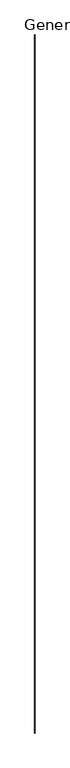
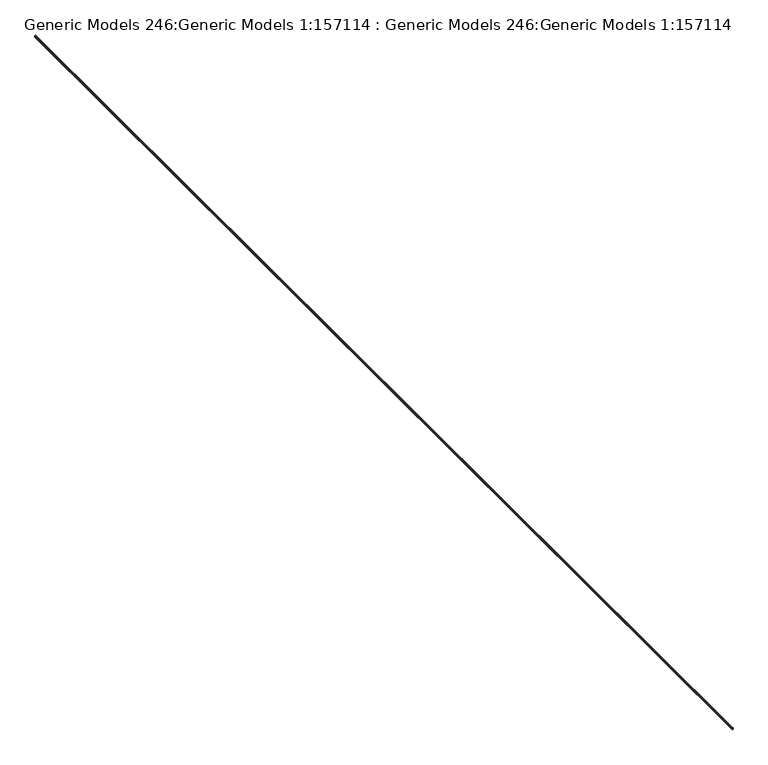
"""IFC4 building model written with IfcOpenShell, lengths in millimetres: proxy geometry, Generic Models 246:Generic Models 1:157114 : Generic Models 246:Generic Models 1:157114."""

from ifc_helpers import new_model, si_unit, point, frame, frame_2d, origin, place, context, project, spatial, polyline, circle_curve, trimmed, segment, composite_curve, outline, extrude, source, transform, mapped, element, save


def generic_models_246_generic_models_1_157114_generic_models_ae619eab(model_context):
    return source(origin(), model_context, "Body", "SweptSolid", [
        extrude(outline(composite_curve([segment(trimmed(circle_curve(frame_2d((6034.2282742, 2076.0989222)), 4.3100275), [point((6037.1430147, 2072.9239222))], [point((6037.1430147, 2079.2739222))], True, "CARTESIAN"), True, "CONTINUOUS"), segment(polyline([(6037.1430147, 2079.2739222), (6040.3180147, 2079.2739222)]), True, "CONTINUOUS"), segment(trimmed(circle_curve(frame_2d((6037.4032742, 2076.0989222)), 4.3100275), [point((6040.3180147, 2079.2739222))], [point((6041.269774, 2078.0032636))], False, "CARTESIAN"), True, "CONTINUOUS"), segment(polyline([(6041.269774, 2078.0032636), (6041.9750492, 2078.5060865), (6042.8263165, 2078.8957455), (6043.7835566, 2079.1539221), (6044.8017683, 2079.2684792), (6045.8330843, 2079.2340312), (6046.829021, 2079.0521977), (6047.7427582, 2078.7315268), (6048.5313398, 2078.2870936), (6049.1576935, 2077.7397917), (6049.8149455, 2075.7547189), (6049.1576935, 2074.4580526), (6048.5313398, 2073.9107507), (6047.7427582, 2073.4663175), (6046.829021, 2073.1456466), (6045.8330843, 2072.9638131), (6044.8017683, 2072.9293651), (6043.7835566, 2073.0439222), (6042.8263165, 2073.3020988), (6041.9750492, 2073.6917578), (6041.269774, 2074.1945807)]), True, "CONTINUOUS"), segment(trimmed(circle_curve(frame_2d((6037.4032742, 2076.0989222)), 4.3100275), [point((6041.269774, 2074.1945807))], [point((6040.3180147, 2072.9239222))], False, "CARTESIAN"), True, "CONTINUOUS"), segment(polyline([(6040.3180147, 2072.9239222), (6037.1430147, 2072.9239222)]), True, "CONTINUOUS")], self_intersect=False)), frame((0.0, 496.8218843, 0.0), z_axis=(0.0, 1.0, 0.0), x_axis=(0.0, 0.0, 1.0)), (0.0, 0.0, 1.0), 7886.7),
    ])


if __name__ == "__main__":
    model = new_model("IFC4")
    model_context = context("Model", 3, world=origin())
    ifc_project = project(units=[si_unit("LENGTHUNIT", "METRE", prefix="MILLI")], contexts=[model_context])
    site = spatial("IfcSite", under=ifc_project)
    building = spatial("IfcBuilding", under=site)
    placement = place(None, origin())
    generic_models_246_generic_models_1_157114_generic_models_shape = generic_models_246_generic_models_1_157114_generic_models_ae619eab(model_context)
    element("IfcBuildingElementProxy", 1, Name="Generic Models 246:Generic Models 1:157114 : Generic Models 246:Generic Models 1:157114", ObjectType="Generic Models 246:Generic Models 1:157114 : Generic Models 246:Generic Models 1:157114", at=placement, inside=building, context=model_context, shape_type="MappedRepresentation", body=[
        mapped(generic_models_246_generic_models_1_157114_generic_models_shape, transform((0.0, 0.0, 0.0), x_axis=(1.0, 0.0, 0.0), y_axis=(0.0, 1.0, 0.0), z_axis=(0.0, 0.0, 1.0))),
    ])
    save(model, "model.ifc")

# Revit data of these elements
# Type "Generic Models 246:Generic Models 1:157114 : Generic Models 246:Generic Models 1:157114"
#   NameOverride = "Generic Models 246:Generic Models 1:157114"
#   ObjectTypeOverride = "Generic Models 246:Generic Models 1"
#   Reference = "Generic Models 1"
#   Category = "Generic Models"
#   Tag = "157114"
# Element 1 (IfcBuildingElementProxy, "Generic Models 246:Generic Models 1:157114 : Generic Models 246:Generic Models 1:157114")
#   Materials on its faces: "_SEALANT AND BACKROD, IF NECESSARY 12051"
# Materials
#   "_SEALANT AND BACKROD, IF NECESSARY 12051": class "Unassigned", colour RGB 190 220 196, transparency 0
